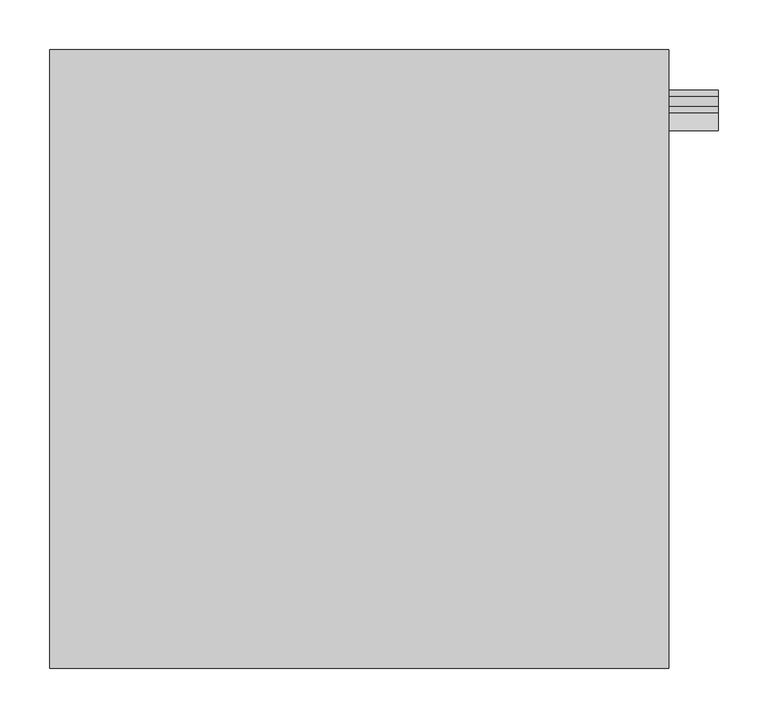
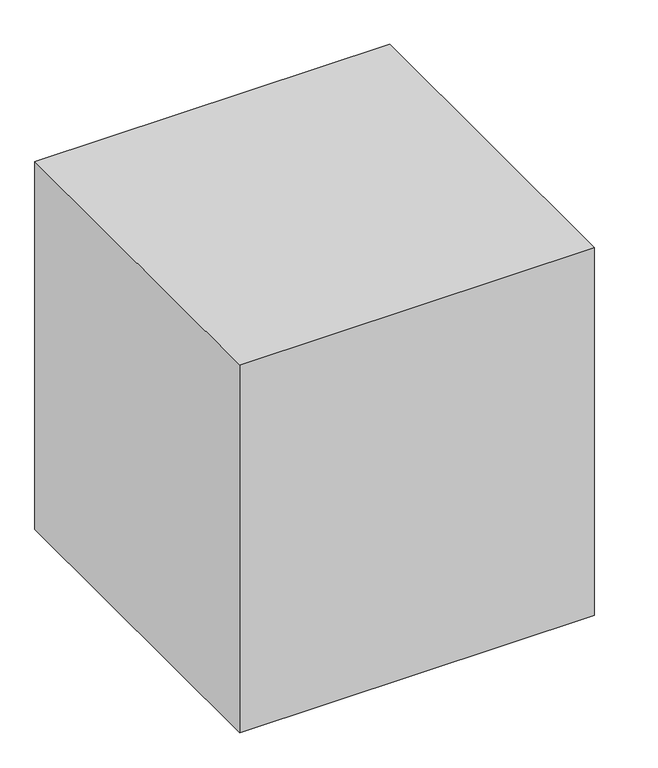
"""IFC4 building model written with IfcOpenShell, lengths in millimetres: proxy geometry, Evaporator coil : Evaporator coil."""

from ifc_helpers import new_model, si_unit, point, frame, frame_2d, origin, origin_with_axes, place, context, project, spatial, polyline, circle_curve, trimmed, segment, composite_curve, outline, extrude, source, transform, mapped, element, save


def mechanical_equipment_1ffd6ebc(model_context):
    return source(origin(), model_context, "Body", "SweptSolid", [
        extrude(outline(composite_curve([segment(trimmed(circle_curve(frame_2d((259.15, 455.6)), 4.8), [point((254.35, 455.6))], [point((263.95, 455.6))], False, "CARTESIAN"), True, "CONTINUOUS"), segment(trimmed(circle_curve(frame_2d((259.15, 455.6)), 4.8), [point((263.95, 455.6))], [point((254.35, 455.6))], False, "CARTESIAN"), True, "CONTINUOUS")], self_intersect=False)), frame((311.15, 0.0, 0.0), z_axis=(1.0, 0.0, 0.0), x_axis=(0.0, 1.0, 0.0)), (0.0, 0.0, 1.0), 50.0),
        extrude(outline(composite_curve([segment(trimmed(circle_curve(frame_2d((259.15, 365.6)), 11.1), [point((248.05, 365.6))], [point((270.25, 365.6))], False, "CARTESIAN"), True, "CONTINUOUS"), segment(trimmed(circle_curve(frame_2d((259.15, 365.6)), 11.1), [point((270.25, 365.6))], [point((248.05, 365.6))], False, "CARTESIAN"), True, "CONTINUOUS")], self_intersect=False)), frame((311.15, 0.0, 0.0), z_axis=(1.0, 0.0, 0.0), x_axis=(0.0, 1.0, 0.0)), (0.0, 0.0, 1.0), 50.0),
        extrude(outline(composite_curve([segment(trimmed(circle_curve(frame_2d((239.15, 35.0)), 9.5), [point((229.65, 35.0))], [point((248.65, 35.0))], False, "CARTESIAN"), True, "CONTINUOUS"), segment(trimmed(circle_curve(frame_2d((239.15, 35.0)), 9.5), [point((248.65, 35.0))], [point((229.65, 35.0))], False, "CARTESIAN"), True, "CONTINUOUS")], self_intersect=False)), frame((311.15, 0.0, 0.0), z_axis=(1.0, 0.0, 0.0), x_axis=(0.0, 1.0, 0.0)), (0.0, 0.0, 1.0), 50.0),
        extrude(outline(polyline([(311.15, 311.15), (311.15, -311.15), (-311.15, -311.15), (-311.15, 311.15), (311.15, 311.15)])), origin_with_axes(), (0.0, 0.0, 1.0), 682.6),
    ])


if __name__ == "__main__":
    model = new_model("IFC4")
    model_context = context("Model", 3, world=origin())
    ifc_project = project(units=[si_unit("LENGTHUNIT", "METRE", prefix="MILLI")], contexts=[model_context])
    site = spatial("IfcSite", under=ifc_project)
    building = spatial("IfcBuilding", under=site)
    placement = place(None, origin())
    mechanical_equipment_shape = mechanical_equipment_1ffd6ebc(model_context)
    element("IfcBuildingElementProxy", 1, Name="Evaporator coil : Evaporator coil", ObjectType="Evaporator coil : Evaporator coil", at=placement, inside=building, context=model_context, shape_type="MappedRepresentation", body=[
        mapped(mechanical_equipment_shape, transform((0.0, 0.0, 0.0), x_axis=(1.0, 0.0, 0.0), y_axis=(0.0, 1.0, 0.0), z_axis=(0.0, 0.0, 1.0))),
    ])
    save(model, "model.ifc")

# Revit data of these elements
# Type "Evaporator coil : Evaporator coil"
#   Type Mark = "EVC-01"
#   Refrigerent = "R410"
#   Width = 2' - 0 1/2"
#   Suction line size = 0' - 0.87402"
#   Length = 2' - 0 1/2"
#   Height = 2' - 2.87402"
#   Drain Dia = 0' - 0.74803"
#   Coil pressure drop = 0.00 in-wg
